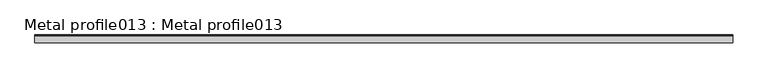
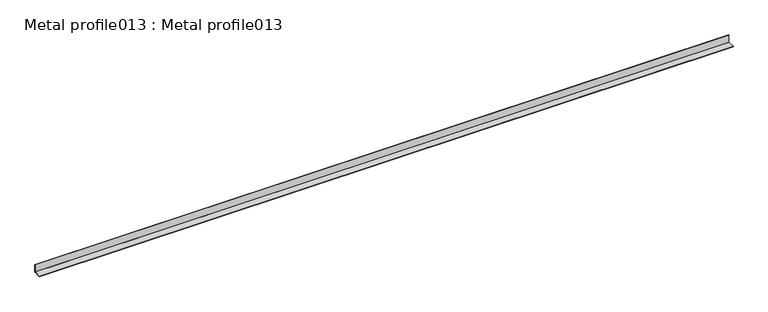
"""IFC4 building model written with IfcOpenShell, lengths in millimetres: proxy geometry, Metal profile013 : Metal profile013."""

from ifc_helpers import new_model, si_unit, point, frame, frame_2d, origin, place, context, project, spatial, polyline, circle_curve, trimmed, segment, composite_curve, outline, extrude, source, transform, mapped, element, save


def metal_profile013_metal_profile013_968b8e9d(model_context):
    return source(origin(), model_context, "Body", "SweptSolid", [
        extrude(outline(composite_curve([segment(polyline([(-4237.2648904, 42605.6253714), (-4235.9848904, 42605.6253714), (-4235.9848904, 42584.7224617)]), True, "CONTINUOUS"), segment(trimmed(circle_curve(frame_2d((-4236.6248904, 42583.8321875)), 1.0964434), [point((-4235.9848904, 42584.7224617))], [point((-4237.5151646, 42583.1921875))], False, "CARTESIAN"), True, "CONTINUOUS"), segment(polyline([(-4237.5151646, 42583.1921875), (-4258.4180743, 42583.1921875), (-4258.4180743, 42584.4721875), (-4237.2648904, 42584.4721875), (-4237.2648904, 42605.6253714)]), True, "CONTINUOUS")], self_intersect=False)), frame((12383.0178845, 0.0, 0.0), z_axis=(1.0, 0.0, 0.0), x_axis=(0.0, 1.0, 0.0)), (0.0, 0.0, 1.0), 2000.0),
    ])


if __name__ == "__main__":
    model = new_model("IFC4")
    model_context = context("Model", 3, world=origin())
    ifc_project = project(units=[si_unit("LENGTHUNIT", "METRE", prefix="MILLI")], contexts=[model_context])
    site = spatial("IfcSite", under=ifc_project)
    building = spatial("IfcBuilding", under=site)
    placement = place(None, origin())
    metal_profile013_metal_profile013_shape = metal_profile013_metal_profile013_968b8e9d(model_context)
    element("IfcBuildingElementProxy", 1, Name="Metal profile013 : Metal profile013", ObjectType="Metal profile013 : Metal profile013", at=placement, inside=building, context=model_context, shape_type="MappedRepresentation", body=[
        mapped(metal_profile013_metal_profile013_shape, transform((0.0, 0.0, 0.0), x_axis=(1.0, 0.0, 0.0), y_axis=(0.0, 1.0, 0.0), z_axis=(0.0, 0.0, 1.0))),
    ])
    save(model, "model.ifc")

# Revit data of these elements
# Type "Metal profile013 : Metal profile013"
#   NameOverride = "Metal profile013"
# Element 1 (IfcBuildingElementProxy, "Metal profile013 : Metal profile013")
#   Materials on its faces: "CORNER BEAD"
# Materials
#   "CORNER BEAD": class "Unassigned", colour RGB 255 241 0, transparency 0
